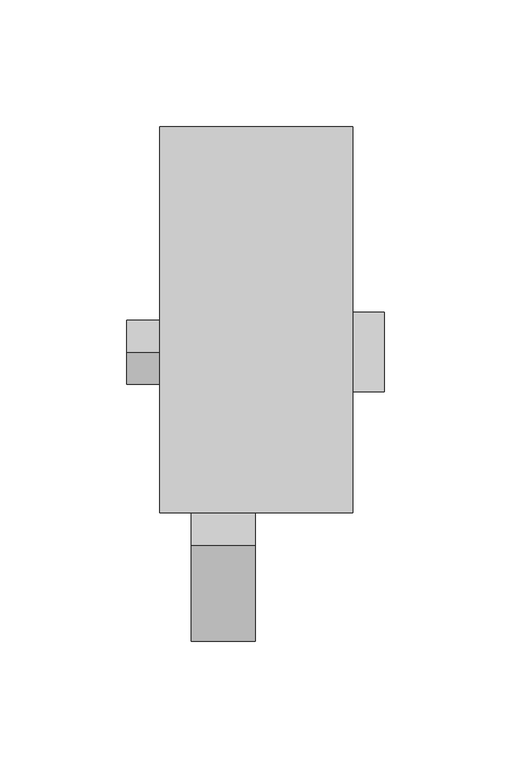
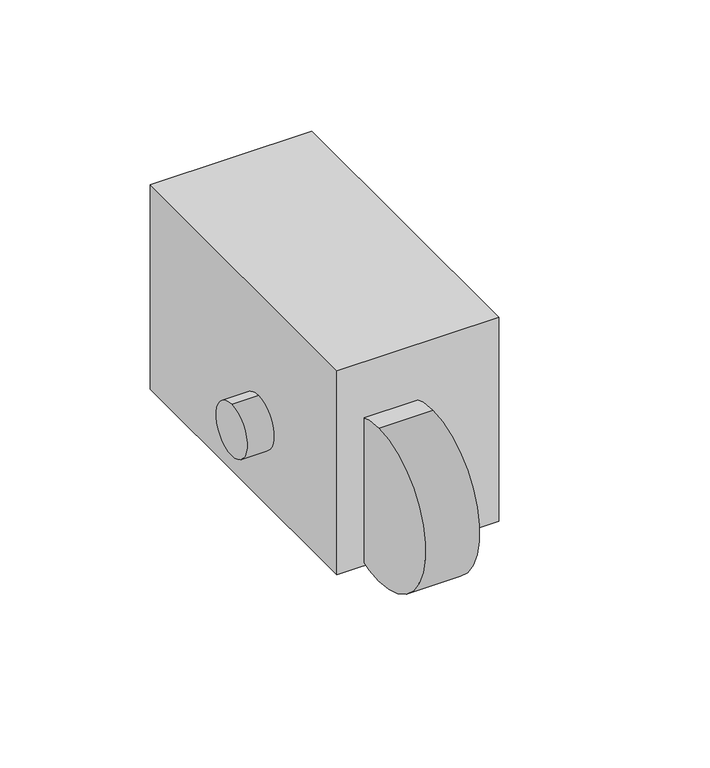
"""IFC4 building model written with IfcOpenShell, lengths in millimetres: proxy geometry, M0765 - Regulator, Vacuum : M0765 - Regulator, Vacuum."""

import ifcopenshell
import ifcopenshell.guid

model = None  # the IFC model being written
_history = None  # IfcOwnerHistory: only IFC2X3 demands one
_inside = {}  # id of a spatial element -> (the spatial element, [elements in it])
_under = {}  # id of a project, library or spatial element -> (it, [spatial elements below it])
_declared = {}  # id of a project -> (the project, [libraries it declares])
_typed = {}  # id of a type object -> (the type object, [elements of that type])
_made_of = {}  # id of a material, layer set ... -> (it, [elements and type objects made of it])


def new_model(schema):
    """Start an empty IFC model of exactly this schema.

    Asked for "IFC4X3", IfcOpenShell would pick the latest addendum, in which some entities
    have other attributes; the version numbers below select the first issue.
    IFC2X3 requires an IfcOwnerHistory on every rooted entity: one is made here for all.
    """
    global model, _history
    if schema == "IFC4X3":
        model = ifcopenshell.file(schema_version=(4, 3, 0, 0))
    else:
        model = ifcopenshell.file(schema=schema)
    _inside.clear()
    _under.clear()
    _declared.clear()
    _typed.clear()
    _made_of.clear()
    _history = None
    if model.schema == "IFC2X3":
        org = make("IfcOrganization", Name="unknown")
        user = make(
            "IfcPersonAndOrganization",
            ThePerson=make("IfcPerson", FamilyName="unknown"),
            TheOrganization=org,
        )
        app = make(
            "IfcApplication",
            ApplicationDeveloper=org,
            Version="unknown",
            ApplicationFullName="unknown",
            ApplicationIdentifier="unknown",
        )
        _history = make(
            "IfcOwnerHistory",
            OwningUser=user,
            OwningApplication=app,
            ChangeAction="ADDED",
            CreationDate=0,
        )
    return model


def make(cls, **values):
    """One entity of the class cls with the attributes given. An attribute that is None is left unset."""
    return model.create_entity(
        cls, **{name: value for name, value in values.items() if value is not None}
    )


def rooted(cls, **values):
    """An entity with a GlobalId (a new one), such as an element, a storey or a relation."""
    return make(cls, GlobalId=ifcopenshell.guid.new(), OwnerHistory=_history, **values)


def si_unit(unit_type, name, prefix=None):
    """IfcSIUnit, for example si_unit("LENGTHUNIT", "METRE", prefix="MILLI")."""
    return make("IfcSIUnit", UnitType=unit_type, Prefix=prefix, Name=name)


def assignment(units):
    """IfcUnitAssignment: the units of a project."""
    return None if units is None else make("IfcUnitAssignment", Units=units)


def point(xyz):
    """IfcCartesianPoint."""
    return None if xyz is None else make("IfcCartesianPoint", Coordinates=xyz)


def direction(xyz):
    """IfcDirection."""
    return None if xyz is None else make("IfcDirection", DirectionRatios=xyz)


def frame(location, z_axis=None, x_axis=None):
    """IfcAxis2Placement3D, a coordinate frame: its origin and axes. An axis left out is left unset."""
    return make(
        "IfcAxis2Placement3D",
        Location=point(location),
        Axis=direction(z_axis),
        RefDirection=direction(x_axis),
    )


def frame_2d(location, x_axis=None):
    """IfcAxis2Placement2D, a coordinate frame in the plane: its origin and x axis."""
    return make(
        "IfcAxis2Placement2D", Location=point(location), RefDirection=direction(x_axis)
    )


def origin():
    """The frame at (0, 0, 0) with its axes left unset."""
    return frame((0.0, 0.0, 0.0))


def origin_with_axes():
    """The frame at (0, 0, 0) with the z axis (0, 0, 1) and the x axis (1, 0, 0) written out."""
    return frame((0.0, 0.0, 0.0), z_axis=(0.0, 0.0, 1.0), x_axis=(1.0, 0.0, 0.0))


def place(relative_to, where):
    """IfcLocalPlacement: puts the frame where relative to a parent placement (None: the world)."""
    return make(
        "IfcLocalPlacement", PlacementRelTo=relative_to, RelativePlacement=where
    )


def context(
    kind, dimensions, precision=None, world=None, true_north=None, identifier=None
):
    """IfcGeometricRepresentationContext, for example the 3D "Model" context."""
    return make(
        "IfcGeometricRepresentationContext",
        ContextIdentifier=identifier,
        ContextType=kind,
        CoordinateSpaceDimension=dimensions,
        Precision=precision,
        WorldCoordinateSystem=world,
        TrueNorth=true_north,
    )


def project(units=None, contexts=None):
    """IfcProject with its units and contexts."""
    return rooted(
        "IfcProject",
        Name="project",
        RepresentationContexts=contexts,
        UnitsInContext=assignment(units),
    )


def spatial(cls, under=None, at=None, **own):
    """A site, building, storey or space (cls), placed at a placement, below another one or the project."""
    s = rooted(cls, ObjectPlacement=at, **own)
    if under is not None:
        _under.setdefault(under.id(), (under, []))[1].append(s)
    return s


def polyline(points):
    """IfcPolyline through the points."""
    return make("IfcPolyline", Points=[point(p) for p in points])


def circle_curve(where, radius):
    """IfcCircle in the frame where."""
    return make("IfcCircle", Position=where, Radius=radius)


def trimmed(basis, trim1, trim2, sense, master):
    """IfcTrimmedCurve: the piece of a basis curve between two trims."""
    return make(
        "IfcTrimmedCurve",
        BasisCurve=basis,
        Trim1=trim1,
        Trim2=trim2,
        SenseAgreement=sense,
        MasterRepresentation=master,
    )


def segment(curve, same_sense, transition):
    """IfcCompositeCurveSegment."""
    return make(
        "IfcCompositeCurveSegment",
        Transition=transition,
        SameSense=same_sense,
        ParentCurve=curve,
    )


def composite_curve(segments, self_intersect=None):
    """IfcCompositeCurve: segments joined end to end."""
    return make("IfcCompositeCurve", Segments=segments, SelfIntersect=self_intersect)


def outline(outer, holes=None, kind="AREA"):
    """IfcArbitraryClosedProfileDef: a profile drawn as a closed curve; with holes, ...WithVoids."""
    if holes is None:
        return make("IfcArbitraryClosedProfileDef", ProfileType=kind, OuterCurve=outer)
    return make(
        "IfcArbitraryProfileDefWithVoids",
        ProfileType=kind,
        OuterCurve=outer,
        InnerCurves=holes,
    )


def extrude(swept, where, along, depth):
    """IfcExtrudedAreaSolid: the profile swept, set in the frame where, extruded along a direction by depth."""
    return make(
        "IfcExtrudedAreaSolid",
        SweptArea=swept,
        Position=where,
        ExtrudedDirection=direction(along),
        Depth=depth,
    )


def shape(context_of_items, identifier, shape_type, items):
    """IfcShapeRepresentation: the items that make up one representation, for example the "Body"."""
    return make(
        "IfcShapeRepresentation",
        ContextOfItems=context_of_items,
        RepresentationIdentifier=identifier,
        RepresentationType=shape_type,
        Items=items,
    )


def source(mapping_origin, context_of_items, identifier, shape_type, items):
    """IfcRepresentationMap: a shape defined once, which mapped items show again and again."""
    return make(
        "IfcRepresentationMap",
        MappingOrigin=mapping_origin,
        MappedRepresentation=shape(context_of_items, identifier, shape_type, items),
    )


def transform(
    local_origin,
    x_axis=None,
    y_axis=None,
    z_axis=None,
    scale=None,
    scale2=None,
    scale3=None,
    uniform=True,
):
    """IfcCartesianTransformationOperator3D, or its non-uniform kind. x_axis, y_axis, z_axis: its Axis1, 2, 3."""
    if uniform:
        return make(
            "IfcCartesianTransformationOperator3D",
            Axis1=direction(x_axis),
            Axis2=direction(y_axis),
            LocalOrigin=point(local_origin),
            Scale=scale,
            Axis3=direction(z_axis),
        )
    return make(
        "IfcCartesianTransformationOperator3DnonUniform",
        Axis1=direction(x_axis),
        Axis2=direction(y_axis),
        LocalOrigin=point(local_origin),
        Scale=scale,
        Axis3=direction(z_axis),
        Scale2=scale2,
        Scale3=scale3,
    )


def mapped(mapping_source, mapping_target):
    """IfcMappedItem: shows the shape of a source again, moved by a transform."""
    return make(
        "IfcMappedItem", MappingSource=mapping_source, MappingTarget=mapping_target
    )


def made_of(thing, what):
    """Note that an element or type object is made of a material, layer set ...; save() writes the relation."""
    if what is not None:
        _made_of.setdefault(what.id(), (what, []))[1].append(thing)
    return thing


def element(
    cls,
    number,
    at=None,
    inside=None,
    cuts=None,
    type_object=None,
    material=None,
    context=None,
    identifier="Body",
    shape_type=None,
    held_by="IfcProductDefinitionShape",
    body=None,
    shapes=None,
    **own,
):
    """One element of the class cls, such as IfcWall. Its Tag is "e" and its number.

    at: its placement. inside: the storey or other place that contains it. cuts: it is an
    opening in that element (IfcRelVoidsElement). A single representation is given by context,
    identifier, shape_type and body (its items); several are given by shapes. held_by: the class
    of the entity that holds the representations. save() writes the other relations.
    """
    e = rooted(cls, Tag="e%d" % number, ObjectPlacement=at, **own)
    if body is not None:
        shapes = [shape(context, identifier, shape_type, body)]
    if shapes is not None:
        e.Representation = make(held_by, Representations=shapes)
    if inside is not None:
        _inside.setdefault(inside.id(), (inside, []))[1].append(e)
    if cuts is not None:
        rooted(
            "IfcRelVoidsElement", RelatingBuildingElement=cuts, RelatedOpeningElement=e
        )
    if type_object is not None:
        _typed.setdefault(type_object.id(), (type_object, []))[1].append(e)
    return made_of(e, material)


def aggregate(whole, parts):
    """IfcRelAggregates: a whole, such as a stair, and the parts it consists of."""
    return rooted("IfcRelAggregates", RelatingObject=whole, RelatedObjects=parts)


def save(model, path):
    """Write the relations noted so far, then the file.

    IfcRelAggregates (storeys below a building ...), IfcRelContainedInSpatialStructure (elements
    in a storey), IfcRelDefinesByType, IfcRelAssociatesMaterial and IfcRelDeclares: one each for
    every whole, place, type object, material and project.
    """
    for whole, parts in _under.values():
        aggregate(whole, parts)
    for where, things in _inside.values():
        rooted(
            "IfcRelContainedInSpatialStructure",
            RelatedElements=things,
            RelatingStructure=where,
        )
    for kind, things in _typed.values():
        rooted("IfcRelDefinesByType", RelatedObjects=things, RelatingType=kind)
    for what, things in _made_of.values():
        rooted("IfcRelAssociatesMaterial", RelatedObjects=things, RelatingMaterial=what)
    for by, libraries in _declared.values():
        rooted("IfcRelDeclares", RelatingContext=by, RelatedDefinitions=libraries)
    model.write(path)


def plane_surface(at):
    """IfcPlane: the flat surface through the origin of the frame at, square to its z axis."""
    return make("IfcPlane", Position=at)


def cylinder_surface(at, radius):
    """IfcCylindricalSurface: all points at the distance radius from the z axis of the frame at."""
    return make("IfcCylindricalSurface", Position=at, Radius=radius)


def revolved_surface(curve, axis_point, axis_direction):
    """IfcSurfaceOfRevolution: the curve turned about the line through axis_point along axis_direction."""
    return make(
        "IfcSurfaceOfRevolution",
        SweptCurve=make("IfcArbitraryOpenProfileDef", ProfileType="CURVE", Curve=curve),
        AxisPosition=make("IfcAxis1Placement", Location=point(axis_point), Axis=direction(axis_direction)),
    )


def advanced_brep(points, edges, surfaces, faces):
    """IfcAdvancedBrep: a solid bounded by faces that lie on surfaces and meet in shared edges.

    An edge is (start, end): straight between two places in points (the first is 0);
    or (start, end, curve); or (start, end, curve, False) where it runs against its curve.
    A face is (place in surfaces, loops), or (place, loops, False) where it looks against
    its surface's normal. A loop lists edges by number (the first is 1), with a minus sign
    where the edge is run from its end to its start. The first loop is the outer one.
    """
    corners = [point(p) for p in points]
    vertices = [make("IfcVertexPoint", VertexGeometry=c) for c in corners]
    made = []
    for start, end, *more in edges:
        made.append(
            make(
                "IfcEdgeCurve",
                EdgeStart=vertices[start],
                EdgeEnd=vertices[end],
                EdgeGeometry=more[0] if more else make("IfcPolyline", Points=[corners[start], corners[end]]),
                SameSense=more[1] if len(more) > 1 else True,
            )
        )
    hull = []
    for where, loops, *sense in faces:
        bounds = []
        for j, loop in enumerate(loops):
            ring = [make("IfcOrientedEdge", EdgeElement=made[abs(k) - 1], Orientation=k > 0) for k in loop]
            bounds.append(
                make(
                    "IfcFaceOuterBound" if j == 0 else "IfcFaceBound",
                    Bound=make("IfcEdgeLoop", EdgeList=ring),
                    Orientation=True,
                )
            )
        hull.append(make("IfcAdvancedFace", Bounds=bounds, FaceSurface=surfaces[where], SameSense=sense[0] if sense else True))
    return make("IfcAdvancedBrep", Outer=make("IfcClosedShell", CfsFaces=hull))


def specialty_equipment_b4fdb6f9(model_context):
    return source(origin(), model_context, "Body", "SolidModel", [
        extrude(outline(polyline([(38.1, -152.4), (-38.1, -152.4), (-38.1, 0.0), (38.1, 0.0), (38.1, -152.4)])), origin_with_axes(), (0.0, 0.0, 1.0), 101.6),
        advanced_brep(
        [(-0.2368425, -76.2, 53.3223414), (-0.2368425, -76.2, 38.1), (-0.2368425, -76.2, 22.8776586), (-0.2368425, -31.8738169, 53.3223414), (-0.2368425, -31.8738169, 22.8776586), (-0.2368425, -31.8738169, 43.8248613), (-0.2368425, -31.8738169, 32.3751387), (-0.2368425, -9.172523, 43.8248613), (-0.2368425, -9.172523, 32.3751387), (-0.2368425, -9.172523, 40.8134652), (-0.2368425, -9.172523, 35.3865348), (-0.2368425, 0.0, 40.8134652), (-0.2368425, 0.0, 35.3865348), (-0.2368425, 0.0, 38.1)],
        [
            (0, 1),
            (1, 2),
            (2, 0, circle_curve(frame((-0.2368425, -76.2, 38.1), z_axis=(0.0, -1.0, 0.0), x_axis=(0.0, 0.0, -1.0)), 15.2223414)),
            (0, 2, circle_curve(frame((-0.2368425, -76.2, 38.1), z_axis=(0.0, -1.0, 0.0), x_axis=(0.0, 0.0, -1.0)), 15.2223414)),
            (3, 0),
            (2, 4),
            (4, 3, circle_curve(frame((-0.2368425, -31.8738169, 38.1), z_axis=(0.0, -1.0, 0.0), x_axis=(0.0, 0.0, -1.0)), 15.2223414)),
            (3, 4, circle_curve(frame((-0.2368425, -31.8738169, 38.1), z_axis=(0.0, -1.0, 0.0), x_axis=(0.0, 0.0, -1.0)), 15.2223414)),
            (5, 3),
            (4, 6),
            (6, 5, circle_curve(frame((-0.2368425, -31.8738169, 38.1), z_axis=(0.0, -1.0, 0.0), x_axis=(0.0, 0.0, -1.0)), 5.7248613)),
            (5, 6, circle_curve(frame((-0.2368425, -31.8738169, 38.1), z_axis=(0.0, -1.0, 0.0), x_axis=(0.0, 0.0, -1.0)), 5.7248613)),
            (7, 5),
            (6, 8),
            (8, 7, circle_curve(frame((-0.2368425, -9.172523, 38.1), z_axis=(0.0, -1.0, 0.0), x_axis=(0.0, 0.0, -1.0)), 5.7248613)),
            (7, 8, circle_curve(frame((-0.2368425, -9.172523, 38.1), z_axis=(0.0, -1.0, 0.0), x_axis=(0.0, 0.0, -1.0)), 5.7248613)),
            (9, 7),
            (8, 10),
            (10, 9, circle_curve(frame((-0.2368425, -9.172523, 38.1), z_axis=(0.0, -1.0, 0.0), x_axis=(0.0, 0.0, -1.0)), 2.7134652)),
            (9, 10, circle_curve(frame((-0.2368425, -9.172523, 38.1), z_axis=(0.0, -1.0, 0.0), x_axis=(0.0, 0.0, -1.0)), 2.7134652)),
            (11, 9),
            (10, 12),
            (12, 11, circle_curve(frame((-0.2368425, 0.0, 38.1), z_axis=(0.0, -1.0, 0.0), x_axis=(0.0, 0.0, -1.0)), 2.7134652)),
            (11, 12, circle_curve(frame((-0.2368425, 0.0, 38.1), z_axis=(0.0, -1.0, 0.0), x_axis=(0.0, 0.0, -1.0)), 2.7134652)),
            (13, 11),
            (12, 13),
        ],
        [
            plane_surface(frame((-0.2368425, -76.2, 38.1), z_axis=(0.0, -1.0, 0.0), x_axis=(0.0, 0.0, -1.0))),
            cylinder_surface(frame((-0.2368425, -1297.7300755, 38.1), z_axis=(0.0, 1.0, 0.0), x_axis=(0.0, 0.0, -1.0)), 15.2223414),
            plane_surface(frame((-0.2368425, -31.8738169, 38.1), z_axis=(0.0, 1.0, 0.0), x_axis=(0.0, 0.0, -1.0))),
            cylinder_surface(frame((-0.2368425, -1297.7300755, 38.1), z_axis=(0.0, 1.0, 0.0), x_axis=(0.0, 0.0, -1.0)), 5.7248613),
            plane_surface(frame((-0.2368425, -9.172523, 38.1), z_axis=(0.0, 1.0, 0.0), x_axis=(0.0, 0.0, -1.0))),
            cylinder_surface(frame((-0.2368425, -1297.7300755, 38.1), z_axis=(0.0, 1.0, 0.0), x_axis=(0.0, 0.0, -1.0)), 2.7134652),
            plane_surface(frame((-0.2368425, 0.0, 38.1), z_axis=(0.0, 1.0, 0.0), x_axis=(0.0, 0.0, -1.0))),
        ],
        [
            (0, [[1, 2, 3]]),
            (0, [[-2, -1, 4]]),
            (1, [[5, -3, 6, 7]]),
            (1, [[-6, -4, -5, 8]]),
            (2, [[9, -7, 10, 11]]),
            (2, [[-10, -8, -9, 12]]),
            (3, [[13, -11, 14, 15]]),
            (3, [[-14, -12, -13, 16]]),
            (4, [[17, -15, 18, 19]]),
            (4, [[-18, -16, -17, 20]]),
            (5, [[21, -19, 22, 23]]),
            (5, [[-22, -20, -21, 24]]),
            (6, [[25, -23, 26]]),
            (6, [[-26, -24, -25]]),
        ],
    ),
        advanced_brep(
        [(50.5631575, -104.5493597, 38.1), (22.2137978, -104.5493597, 38.1), (22.2137978, -73.2506403, 38.1), (50.5631575, -73.2506403, 38.1), (50.5631575, -88.9, 38.1), (-0.2368425, -127.0, 38.1), (-0.2368425, -88.9, 38.1), (-0.2368425, -50.8, 38.1)],
        [
            (0, 1),
            (1, 2, circle_curve(frame((22.2137978, -88.9, 38.1), z_axis=(1.0, 0.0, 0.0), x_axis=(0.0, 1.0, 0.0)), 15.6493597)),
            (2, 3),
            (3, 0, circle_curve(frame((50.5631575, -88.9, 38.1), z_axis=(-1.0, 0.0, 0.0), x_axis=(0.0, 1.0, 0.0)), 15.6493597)),
            (2, 1, circle_curve(frame((22.2137978, -88.9, 38.1), z_axis=(1.0, 0.0, 0.0), x_axis=(0.0, 1.0, 0.0)), 15.6493597)),
            (0, 3, circle_curve(frame((50.5631575, -88.9, 38.1), z_axis=(-1.0, 0.0, 0.0), x_axis=(0.0, 1.0, 0.0)), 15.6493597)),
            (4, 0),
            (3, 4),
            (5, 6),
            (6, 7),
            (7, 5, circle_curve(frame((-0.2368425, -88.9, 38.1), z_axis=(-1.0, 0.0, 0.0), x_axis=(0.0, 1.0, 0.0)), 38.1)),
            (5, 7, circle_curve(frame((-0.2368425, -88.9, 38.1), z_axis=(-1.0, 0.0, 0.0), x_axis=(0.0, 1.0, 0.0)), 38.1)),
            (1, 5),
            (7, 2),
        ],
        [
            cylinder_surface(frame((-51.0368425, -88.9, 38.1), z_axis=(1.0, 0.0, 0.0), x_axis=(0.0, 1.0, 0.0)), 15.6493597),
            plane_surface(frame((50.5631575, -88.9, 38.1), z_axis=(1.0, 0.0, 0.0), x_axis=(0.0, 1.0, 0.0))),
            plane_surface(frame((-0.2368425, -88.9, 38.1), z_axis=(-1.0, 0.0, 0.0), x_axis=(0.0, 1.0, 0.0))),
            revolved_surface(polyline([(-0.2368425, -50.8, 38.1), (22.2137978, -73.2506403, 38.1)]), (-51.0368425, -88.9, 38.1), (1.0, 0.0, 0.0)),
        ],
        [
            (0, [[1, 2, 3, 4]]),
            (0, [[-3, 5, -1, 6]]),
            (1, [[7, -4, 8]]),
            (1, [[-8, -6, -7]]),
            (2, [[9, 10, 11]]),
            (2, [[-10, -9, 12]]),
            (3, [[13, -11, 14, -2]]),
            (3, [[-14, -12, -13, -5]]),
        ],
    ),
        extrude(outline(composite_curve([segment(trimmed(circle_curve(frame_2d((-88.9, 38.1)), 12.7), [point((-88.9, 25.4))], [point((-88.9, 50.8))], False, "CARTESIAN"), True, "CONTINUOUS"), segment(trimmed(circle_curve(frame_2d((-88.9, 38.1)), 12.7), [point((-88.9, 50.8))], [point((-88.9, 25.4))], False, "CARTESIAN"), True, "CONTINUOUS")], self_intersect=False)), frame((-51.0368425, 0.0, 0.0), z_axis=(1.0, 0.0, 0.0), x_axis=(0.0, 1.0, 0.0)), (0.0, 0.0, 1.0), 50.8),
        extrude(outline(composite_curve([segment(polyline([(-69.85, 0.0), (-107.95, 0.0)]), True, "CONTINUOUS"), segment(trimmed(circle_curve(frame_2d((-107.95, 19.05)), 19.05), [point((-107.95, 0.0))], [point((-127.0, 19.05))], False, "CARTESIAN"), True, "CONTINUOUS"), segment(polyline([(-127.0, 19.05), (-127.0, 57.15)]), True, "CONTINUOUS"), segment(trimmed(circle_curve(frame_2d((-107.95, 57.15)), 19.05), [point((-127.0, 57.15))], [point((-107.95, 76.2))], False, "CARTESIAN"), True, "CONTINUOUS"), segment(polyline([(-107.95, 76.2), (-69.85, 76.2)]), True, "CONTINUOUS"), segment(trimmed(circle_curve(frame_2d((-69.85, 57.15)), 19.05), [point((-69.85, 76.2))], [point((-50.8, 57.15))], False, "CARTESIAN"), True, "CONTINUOUS"), segment(polyline([(-50.8, 57.15), (-50.8, 19.05)]), True, "CONTINUOUS"), segment(trimmed(circle_curve(frame_2d((-69.85, 19.05)), 19.05), [point((-50.8, 19.05))], [point((-69.85, 0.0))], False, "CARTESIAN"), True, "CONTINUOUS")], self_intersect=False)), frame((-25.6368425, 0.0, 0.0), z_axis=(1.0, 0.0, 0.0), x_axis=(0.0, 1.0, 0.0)), (0.0, 0.0, 1.0), 25.4),
        extrude(outline(composite_curve([segment(trimmed(circle_curve(frame_2d((-165.1, 38.1)), 38.1), [point((-165.1, 0.0))], [point((-165.1, 76.2))], False, "CARTESIAN"), True, "CONTINUOUS"), segment(trimmed(circle_curve(frame_2d((-165.1, 38.1)), 38.1), [point((-165.1, 76.2))], [point((-165.1, 0.0))], False, "CARTESIAN"), True, "CONTINUOUS")], self_intersect=False)), frame((-25.6368425, 0.0, 0.0), z_axis=(1.0, 0.0, 0.0), x_axis=(0.0, 1.0, 0.0)), (0.0, 0.0, 1.0), 25.4),
    ])


if __name__ == "__main__":
    model = new_model("IFC4")
    model_context = context("Model", 3, world=origin())
    ifc_project = project(units=[si_unit("LENGTHUNIT", "METRE", prefix="MILLI")], contexts=[model_context])
    site = spatial("IfcSite", under=ifc_project)
    building = spatial("IfcBuilding", under=site)
    placement = place(None, origin())
    specialty_equipment_shape = specialty_equipment_b4fdb6f9(model_context)
    element("IfcBuildingElementProxy", 1, Name="M0765 - Regulator, Vacuum : M0765 - Regulator, Vacuum", ObjectType="M0765 - Regulator, Vacuum : M0765 - Regulator, Vacuum", at=placement, inside=building, context=model_context, shape_type="MappedRepresentation", body=[
        mapped(specialty_equipment_shape, transform((0.0, 0.0, 0.0), x_axis=(1.0, 0.0, 0.0), y_axis=(0.0, 1.0, 0.0), z_axis=(0.0, 0.0, 1.0))),
    ])
    save(model, "model.ifc")

# Revit data of these elements
# Type "M0765 - Regulator, Vacuum : M0765 - Regulator, Vacuum"
#   Watts2 = "0"
#   Watts1 = "0"
#   Unit_Issue = "EA"
#   UTIL_6_Misc = "-"
#   UTIL_5_NonMedGas = "-"
#   UTIL_4_MiscGas = "-"
#   UTIL_3_MedGas = "B"
#   UTIL_2_Elec = "-"
#   UTIL_1_WaterDrain = "-"
#   Nomenclature = "Regulator, Vacuum"
#   NSN = "6515"
#   Location [instance default] = ""
#   JSN = "M0765"
#   Fund_Source_VA = "-"
#   Fund_Source_Navy = "-"
#   Fund_Source_Army = "-"
#   Fund_Source_AF = "-"
#   ELEC_Volts2 = "0"
#   ELEC_Volts1 = "0"
#   ELEC_Phase2 = "0"
#   ELEC_Phase1 = "0"
#   ELEC_HertzSwitch = "0"
#   ELEC_HertzDependent = "0"
#   ELEC_Hertz = "0"
#   ELEC_Amps2 = "0"
#   ELEC_Amps1 = "0"
#   DetailDescription = "Vacuum pressure regulator for connection to central piped vacuum system. Standard display scale is graduated at least from 0 to 200 mm Hg of vacuum. Displays on specialized regulators may cover other vacuum ranges. Regulator type (continuous, intermittent, continuous/intermittent, surgical, pediatric, thoracic, etc.) as required. To be used in delivery, neonatal, pediatrics or any area where suction is required. Database pricing reflects continuous regulators graduated to 200 mm Hg with a full line vacuum selection switch and DISS configured inlets and outlets."
#   CAT_VA = "C"
#   CAT_Navy = "C"
#   CAT_IHS = "-"
#   CAT_Army = "C"
#   CAT_AF = "C"
#   BTUperhour = "0"
#   Weight_IP = 1
#   Default Elevation = 4' - 0"
#   DIM_Width_IP = 0' - 3"
#   DIM_Height_IP = 0' - 6"
#   DIM_Depth_IP = 0' - 4"
#   finish [instance default] = none
# Element 1 (IfcBuildingElementProxy, "M0765 - Regulator, Vacuum : M0765 - Regulator, Vacuum")
#   Location = "LDAT1"
#   Materials on its faces: "EquipSpace"
# Materials
#   "EquipSpace": class "Unassigned", colour RGB 221 217 195, transparency 0.5
